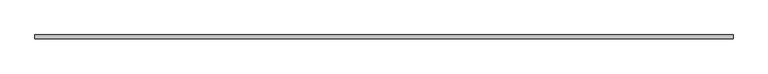
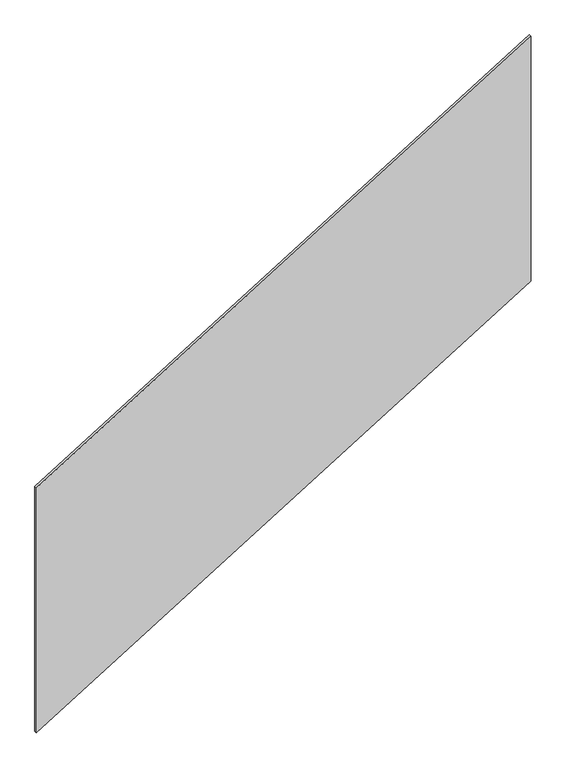
"""IFC4 building model written with IfcOpenShell, lengths in millimetres: railing geometry, ML_Guarda_corpo lance : ML_Guarda_corpo lance."""

from ifc_helpers import new_model, si_unit, frame, origin, place, context, project, spatial, polyline, outline, extrude, source, transform, mapped, element, save


def railing_c44cfcee(model_context):
    return source(origin(), model_context, "Body", "SweptSolid", [
        extrude(outline(polyline([(1672.2222222, -4460.281307), (500.0, -4460.281307), (1877.7777778, -2220.281307), (3050.0, -2220.281307), (1672.2222222, -4460.281307)])), frame((0.0, -5573.3699847, 0.0), z_axis=(0.0, 1.0, 0.0), x_axis=(0.0, 0.0, 1.0)), (0.0, 0.0, 1.0), 12.0),
    ])


if __name__ == "__main__":
    model = new_model("IFC4")
    model_context = context("Model", 3, world=origin())
    ifc_project = project(units=[si_unit("LENGTHUNIT", "METRE", prefix="MILLI")], contexts=[model_context])
    site = spatial("IfcSite", under=ifc_project)
    building = spatial("IfcBuilding", under=site)
    placement = place(None, origin())
    railing_shape = railing_c44cfcee(model_context)
    element("IfcRailing", 1, ObjectType="ML_Guarda_corpo lance : ML_Guarda_corpo lance", at=placement, inside=building, context=model_context, shape_type="MappedRepresentation", body=[
        mapped(railing_shape, transform((0.0, 0.0, 0.0), x_axis=(1.0, 0.0, 0.0), y_axis=(0.0, 1.0, 0.0), z_axis=(0.0, 0.0, 1.0))),
    ])
    save(model, "model.ifc")

# Revit data of these elements
# Type "ML_Guarda_corpo lance : ML_Guarda_corpo lance"
#   ME_Área = 2.62578 m²
#   ME_Espessura [instance default] = 0.012 m
#   ME_Compr Painéis = 2.629804 m
#   ME_Altura = 0.998469 m
#   ME_Material Tipo Vidro [instance default] = .VIDRO GENÉRICO
# Element 1 (IfcRailing, "ML_Guarda_corpo lance : ML_Guarda_corpo lance")
#   Materials on its faces: ".VIDRO GENÉRICO"
# Materials
#   ".VIDRO GENÉRICO": class ".CC_VIDRO", colour RGB 0 128 192, transparency 0.9, Description = "Vidro comum", Cost = 0
